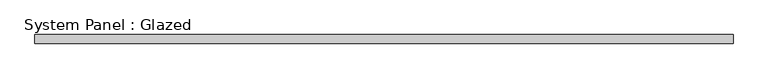
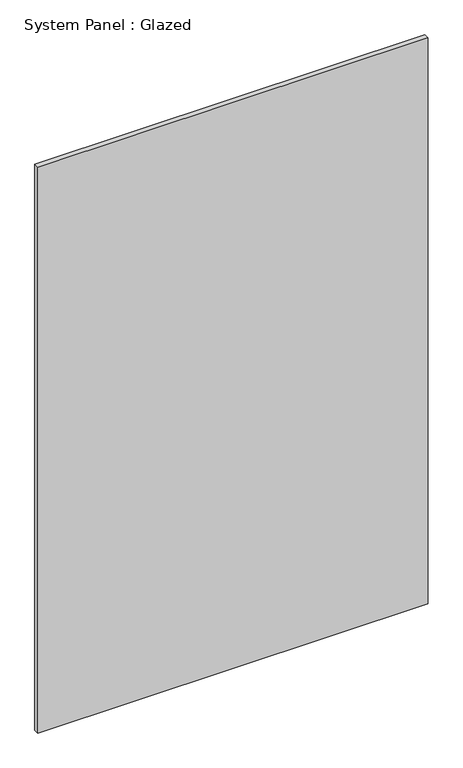
"""IFC4 building model written with IfcOpenShell, lengths in millimetres: plate geometry, System Panel : Glazed."""

from ifc_helpers import new_model, si_unit, origin, origin_with_axes, place, context, project, spatial, polyline, outline, extrude, source, transform, mapped, element, save


def system_panel_glazed_a9dfd4e8(model_context):
    return source(origin(), model_context, "Body", "SweptSolid", [
        extrude(outline(polyline([(962.5000001, 24.5), (-962.5000001, 24.5), (-962.5000001, 49.5), (962.5000001, 49.5), (962.5000001, 24.5)])), origin_with_axes(), (0.0, 0.0, 1.0), 2950.0),
    ])


if __name__ == "__main__":
    model = new_model("IFC4")
    model_context = context("Model", 3, world=origin())
    ifc_project = project(units=[si_unit("LENGTHUNIT", "METRE", prefix="MILLI")], contexts=[model_context])
    site = spatial("IfcSite", under=ifc_project)
    building = spatial("IfcBuilding", under=site)
    placement = place(None, origin())
    system_panel_glazed_shape = system_panel_glazed_a9dfd4e8(model_context)
    element("IfcPlate", 1, ObjectType="System Panel : Glazed", at=placement, inside=building, context=model_context, shape_type="MappedRepresentation", body=[
        mapped(system_panel_glazed_shape, transform((0.0, 0.0, 0.0), x_axis=(1.0, 0.0, 0.0), y_axis=(0.0, 1.0, 0.0), z_axis=(0.0, 0.0, 1.0))),
    ])
    save(model, "model.ifc")

# Revit data of these elements
# Element 1 (IfcPlate, "System Panel : Glazed")
#   Materials on its faces: "Glass"
# Materials
#   "Glass": class "Glass", colour RGB 0 128 192, transparency 0.9
